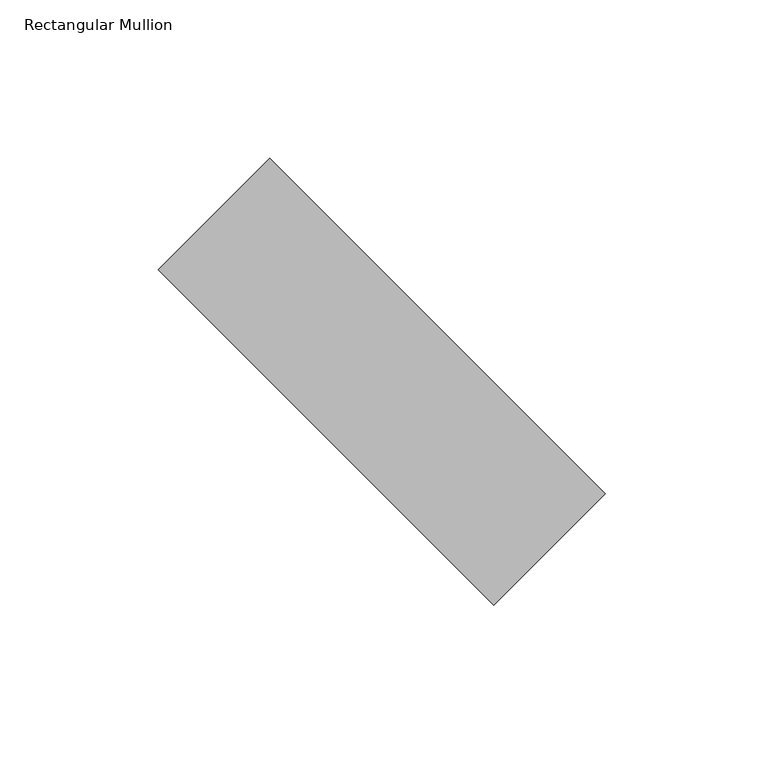
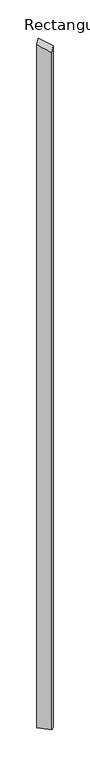
"""IFC4 building model written with IfcOpenShell, lengths in millimetres: member geometry, Rectangular Mullion : tilted mullions."""

from ifc_helpers import new_model, si_unit, origin, place, context, project, spatial, faceted_brep, source, transform, mapped, element, save


def rectangular_mullion_7177dd57(model_context):
    return source(origin(), model_context, "Body", "Brep", [
        faceted_brep([(-35.3553391, 70.7106781, -7999.2401644), (70.7106781, -35.3553391, -7999.2401644), (35.3553391, -70.7106781, -7999.2401644), (-70.7106781, 35.3553391, -7999.2401644), (-70.7106781, 35.3553391, 10.0207535), (-35.3553391, 70.7106781, 55.0681747), (35.3553391, -70.7106781, -55.0681747), (70.7106781, -35.3553391, -10.0207535)], [[[0, 1, 2, 3]], [[4, 5, 0, 3]], [[6, 4, 3, 2]], [[7, 6, 2, 1]], [[5, 7, 1, 0]], [[5, 4, 6, 7]]]),
    ])


if __name__ == "__main__":
    model = new_model("IFC4")
    model_context = context("Model", 3, world=origin())
    ifc_project = project(units=[si_unit("LENGTHUNIT", "METRE", prefix="MILLI")], contexts=[model_context])
    site = spatial("IfcSite", under=ifc_project)
    building = spatial("IfcBuilding", under=site)
    placement = place(None, origin())
    rectangular_mullion_shape = rectangular_mullion_7177dd57(model_context)
    element("IfcMember", 1, ObjectType="Rectangular Mullion : tilted mullions", at=placement, inside=building, context=model_context, shape_type="MappedRepresentation", body=[
        mapped(rectangular_mullion_shape, transform((0.0, 0.0, 0.0), x_axis=(1.0, 0.0, 0.0), y_axis=(0.0, 1.0, 0.0), z_axis=(0.0, 0.0, 1.0))),
    ])
    save(model, "model.ifc")

# Revit data of these elements
# Type "Rectangular Mullion : tilted mullions"
#   built-in parameter 1007304 = 0.492126 (stored number, unit not read)
#   built-in parameter 1007301 = 0.082021 (stored number, unit not read)
#   built-in parameter 1007300 = 0.082021 (stored number, unit not read)
# Element 1 (IfcMember, "Rectangular Mullion : tilted mullions")
#   Materials on its faces: "Aluminum"
# Materials
#   "Aluminum": class "Metal", colour RGB 244 244 244, transparency 0, Description = "Aluminum 6061", Cost = 0
